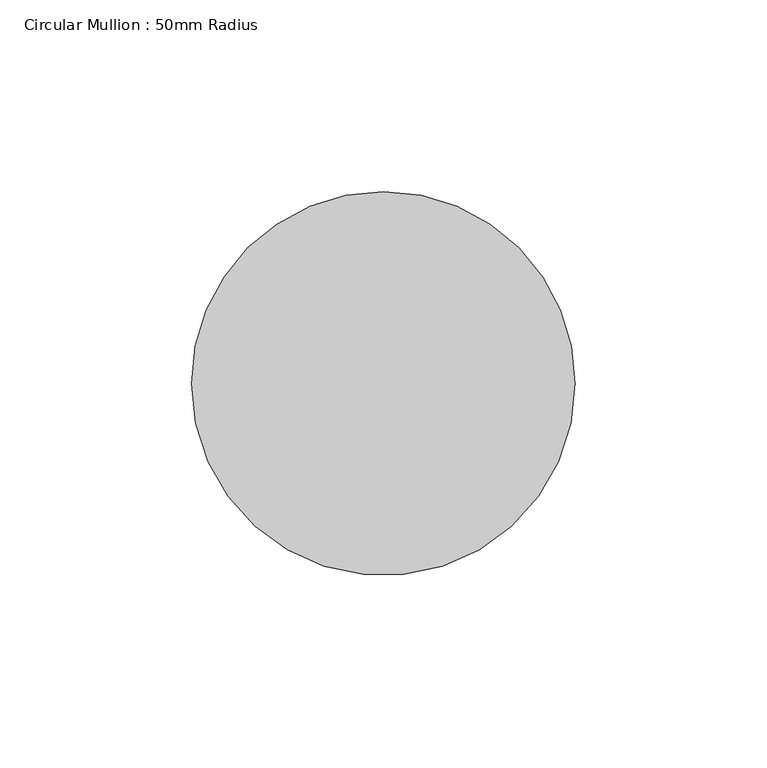
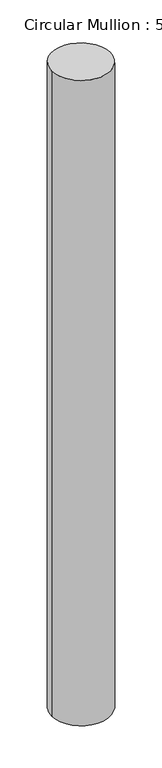
"""IFC4 building model written with IfcOpenShell, lengths in millimetres: member geometry, Circular Mullion : 50mm Radius."""

from ifc_helpers import new_model, si_unit, frame, origin, place, context, project, spatial, ellipse_curve, source, transform, mapped, element, save
from ifc_brep_helpers import plane_surface, cylinder_surface, advanced_brep


def circular_mullion_50mm_radius_68949e39(model_context):
    return source(origin(), model_context, "Body", "AdvancedBrep", [
        advanced_brep(
        [(-100.0, 0.0, 0.8749007), (0.0, 0.0, 0.0), (0.0, 0.0, -1167.3490886), (-100.0, 0.0, -1168.2588755)],
        [
            (0, 1, ellipse_curve(frame((-50.0, 0.0, 0.4374503), z_axis=(-0.00874780865600445, -0.014048852320208432, -0.9998630434175488), x_axis=(-0.5285039150610167, -0.8487695313554682, 0.016549755520753655)), 50.0068488, 50.0)),
            (1, 2),
            (2, 3, ellipse_curve(frame((-50.0, 0.0, -1167.8039821), z_axis=(-0.009096520978293698, -0.014608879192162734, 0.9998519060115055), x_axis=(0.5284980280920648, 0.8487600769697167, 0.017209475446950877)), 50.0074058, 50.0)),
            (3, 0),
            (1, 0, ellipse_curve(frame((-50.0, 0.0, 0.4374503), z_axis=(-0.00874780865600445, -0.014048852320208432, -0.9998630434175488), x_axis=(-0.5285039150610167, -0.8487695313554682, 0.016549755520753655)), 50.0068488, 50.0)),
            (3, 2, ellipse_curve(frame((-50.0, 0.0, -1167.8039821), z_axis=(-0.009096520978293698, -0.014608879192162734, 0.9998519060115055), x_axis=(0.5284980280920648, 0.8487600769697167, 0.017209475446950877)), 50.0074058, 50.0)),
        ],
        [
            cylinder_surface(frame((-50.0, 0.0, 0.0), z_axis=(0.0, 0.0, 1.0), x_axis=(1.0, 0.0, 0.0)), 50.0),
            plane_surface(frame((-258.7403894, 161.1100584, 0.0), z_axis=(0.00874780865600445, 0.014048852320208432, 0.9998630434175488), x_axis=(0.5285039150610162, 0.8487695313554683, -0.016549755520765017))),
            plane_surface(frame((-258.7403894, 161.1100584, -1167.3490886), z_axis=(0.009096520978293698, 0.014608879192162734, -0.9998519060115055), x_axis=(0.5284980280920647, 0.8487600769697168, 0.017209475446966493))),
        ],
        [
            (0, [[1, 2, 3, 4]]),
            (0, [[5, -4, 6, -2]]),
            (1, [[-1, -5]]),
            (2, [[-6, -3]]),
        ],
    ),
    ])


if __name__ == "__main__":
    model = new_model("IFC4")
    model_context = context("Model", 3, world=origin())
    ifc_project = project(units=[si_unit("LENGTHUNIT", "METRE", prefix="MILLI")], contexts=[model_context])
    site = spatial("IfcSite", under=ifc_project)
    building = spatial("IfcBuilding", under=site)
    placement = place(None, origin())
    circular_mullion_50mm_radius_shape = circular_mullion_50mm_radius_68949e39(model_context)
    element("IfcMember", 1, ObjectType="Circular Mullion : 50mm Radius", at=placement, inside=building, context=model_context, shape_type="MappedRepresentation", body=[
        mapped(circular_mullion_50mm_radius_shape, transform((0.0, 0.0, 0.0), x_axis=(1.0, 0.0, 0.0), y_axis=(0.0, 1.0, 0.0), z_axis=(0.0, 0.0, 1.0))),
    ])
    save(model, "model.ifc")

# Revit data of these elements
# Type "Circular Mullion : 50mm Radius"
#   built-in parameter 1007350 = 0.164042 (stored number, unit not read)
# Element 1 (IfcMember, "Circular Mullion : 50mm Radius")
#   Materials on its faces: "Aluminium"
# Materials
#   "Aluminium": class "Metal", colour RGB 247 247 247, transparency 0, Description = "Aluminium 6061", Cost = 0
